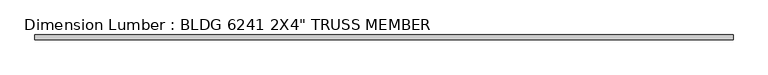
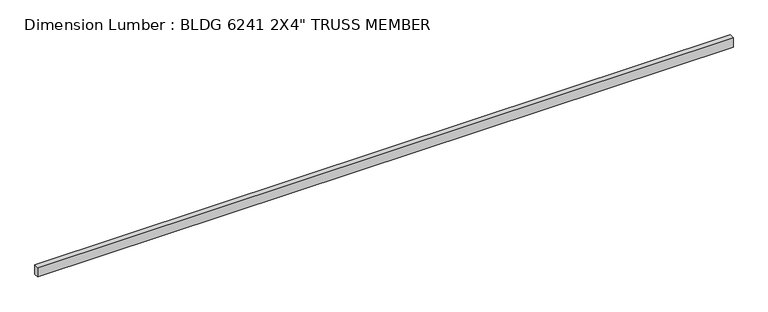
"""IFC4 building model written with IfcOpenShell, lengths in millimetres: beam geometry."""

from ifc_helpers import new_model, si_unit, frame, origin, place, context, project, spatial, polyline, outline, extrude, source, transform, mapped, element, save


def beam_38f3c654(model_context):
    return source(origin(), model_context, "Body", "SweptSolid", [
        extrude(outline(polyline([(3581.4, 25.4), (3581.4, -25.4), (-3556.0, -25.4), (-3556.0, 25.4), (3581.4, 25.4)])), frame((0.0, 0.0, -50.8), z_axis=(0.0, 0.0, 1.0), x_axis=(1.0, 0.0, 0.0)), (0.0, 0.0, 1.0), 101.6),
    ])


if __name__ == "__main__":
    model = new_model("IFC4")
    model_context = context("Model", 3, world=origin())
    ifc_project = project(units=[si_unit("LENGTHUNIT", "METRE", prefix="MILLI")], contexts=[model_context])
    site = spatial("IfcSite", under=ifc_project)
    building = spatial("IfcBuilding", under=site)
    placement = place(None, origin())
    beam_shape = beam_38f3c654(model_context)
    element("IfcBeam", 1, ObjectType="Dimension Lumber : BLDG 6241 2X4\" TRUSS MEMBER", at=placement, inside=building, context=model_context, shape_type="MappedRepresentation", body=[
        mapped(beam_shape, transform((0.0, 0.0, 0.0), x_axis=(1.0, 0.0, 0.0), y_axis=(0.0, 1.0, 0.0), z_axis=(0.0, 0.0, 1.0))),
    ])
    save(model, "model.ifc")

# Revit data of these elements
# Type "Dimension Lumber : BLDG 6241 2X4\" TRUSS MEMBER"
#   Assembly Code = "B10"
#   A = 0.273472 SF
#   Length [instance default] = 5' - 0"
#   b = 0' - 2"
#   d = 0' - 4"
#   Structural Material [instance default] = Softwood, Lumber
# Element 1 (IfcBeam, "Dimension Lumber : BLDG 6241 2X4\" TRUSS MEMBER")
#   Materials on its faces: "Softwood, Lumber"
# Materials
#   "Softwood, Lumber": class "Wood", colour RGB 223 192 134, transparency 0, Description = "Pinus Echinata", Cost = 0
